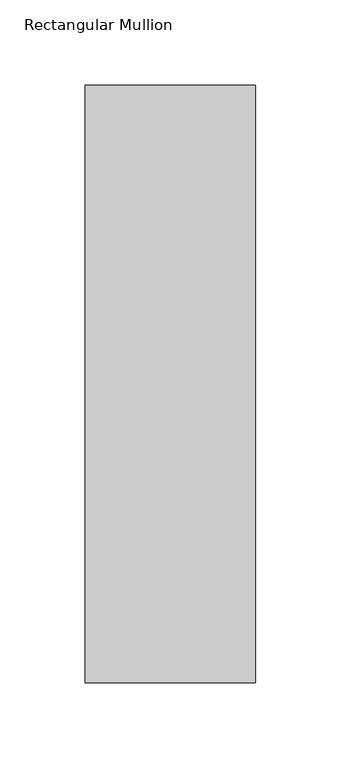
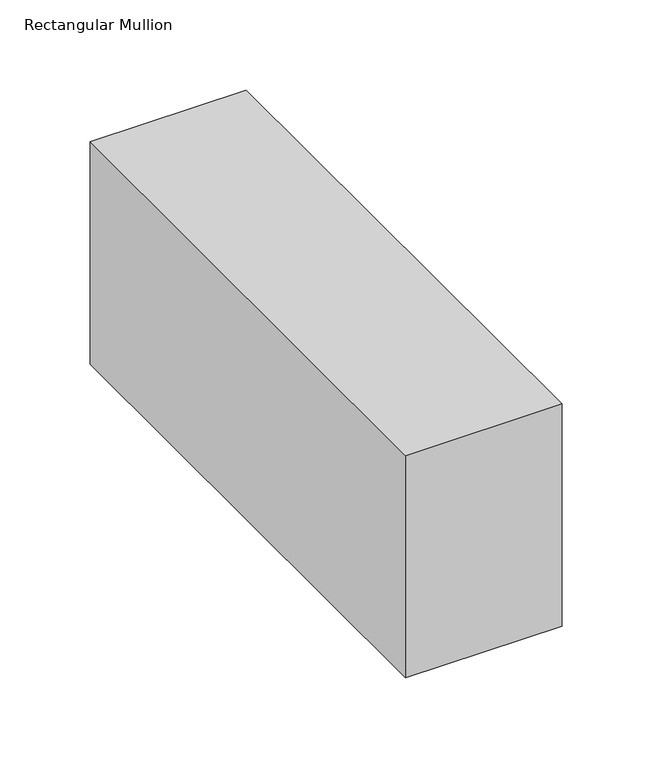
"""IFC4 building model written with IfcOpenShell, lengths in millimetres: member geometry, Rectangular Mullion : WWm-100x350-100mmOffset."""

from ifc_helpers import new_model, si_unit, frame, origin, place, context, project, spatial, polyline, outline, extrude, source, transform, mapped, element, save


def rectangular_mullion_f9ad5075(model_context):
    return source(origin(), model_context, "Body", "SweptSolid", [
        extrude(outline(polyline([(0.0, 175.0), (0.0, -175.0), (-100.0, -175.0), (-100.0, 175.0), (0.0, 175.0)])), frame((0.0, 0.0, -150.381466), z_axis=(0.0, 0.0, 1.0), x_axis=(1.0, 0.0, 0.0)), (0.0, 0.0, 1.0), 150.381466),
    ])


if __name__ == "__main__":
    model = new_model("IFC4")
    model_context = context("Model", 3, world=origin())
    ifc_project = project(units=[si_unit("LENGTHUNIT", "METRE", prefix="MILLI")], contexts=[model_context])
    site = spatial("IfcSite", under=ifc_project)
    building = spatial("IfcBuilding", under=site)
    placement = place(None, origin())
    rectangular_mullion_shape = rectangular_mullion_f9ad5075(model_context)
    element("IfcMember", 1, ObjectType="Rectangular Mullion : WWm-100x350-100mmOffset", at=placement, inside=building, context=model_context, shape_type="MappedRepresentation", body=[
        mapped(rectangular_mullion_shape, transform((0.0, 0.0, 0.0), x_axis=(1.0, 0.0, 0.0), y_axis=(0.0, 1.0, 0.0), z_axis=(0.0, 0.0, 1.0))),
    ])
    save(model, "model.ifc")

# Revit data of these elements
# Type "Rectangular Mullion : WWm-100x350-100mmOffset"
#   built-in parameter 1007304 = 1.14829 (stored number, unit not read)
#   built-in parameter 1007301 = 0.164042 (stored number, unit not read)
#   built-in parameter 1007300 = 0.164042 (stored number, unit not read)
# Element 1 (IfcMember, "Rectangular Mullion : WWm-100x350-100mmOffset")
#   Materials on its faces: "WW-EC-RGB-Mullion"
# Materials
#   "WW-EC-RGB-Mullion": class "Generic", colour RGB 255 255 255, transparency 0, Comments = "If region requests black mullions, switch asset color to RGB 25-25-25", Description = "Generic Color", Cost = 0
